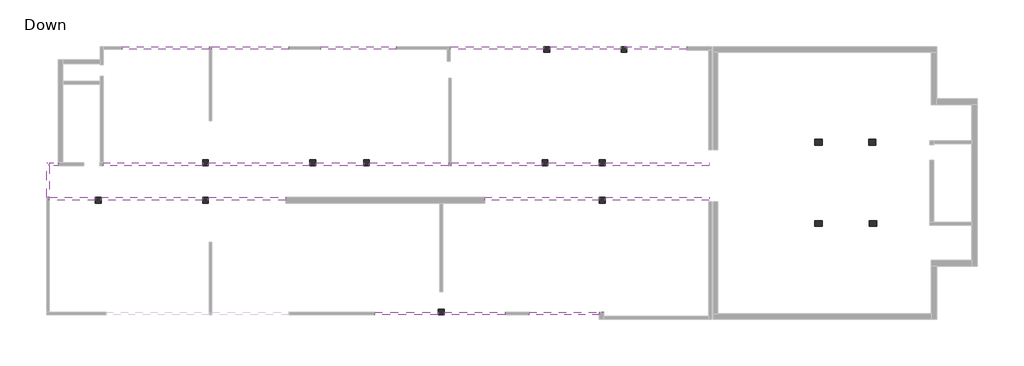
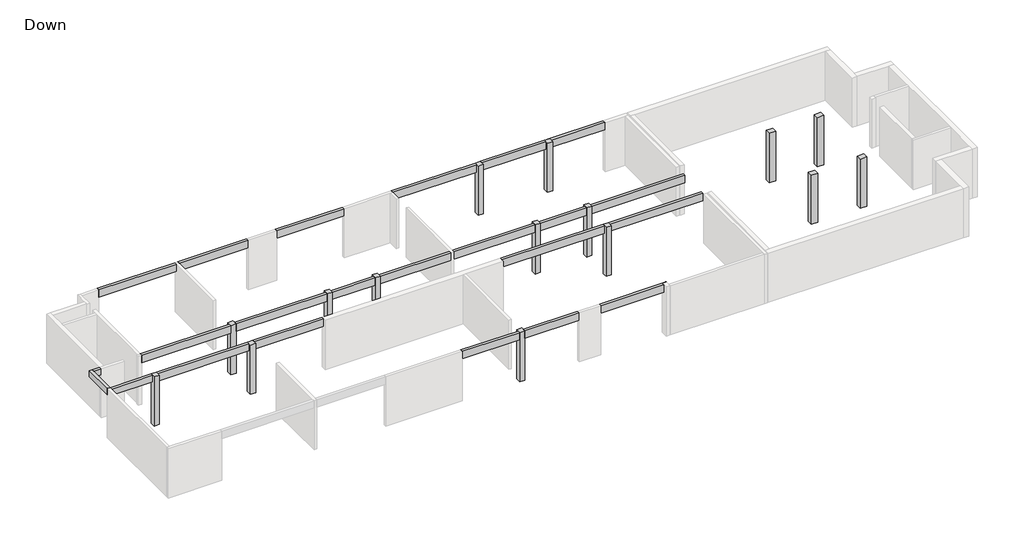
# One storey, part 2 of 2: 23 beams, 15 columns.
"""IFC4 building model written with IfcOpenShell, lengths in millimetres."""

from ifc_helpers import new_model, si_unit, origin, place, context, project, spatial, faceted_brep, element, save

model = new_model("IFC4")

# Units and contexts
model_context = context("Model", 3, world=origin())
ifc_project = project(units=[si_unit("LENGTHUNIT", "METRE", prefix="MILLI")], contexts=[model_context])

# Site, building, storey
site = spatial("IfcSite", under=ifc_project)
building = spatial("IfcBuilding", under=site)
storey = spatial("IfcBuildingStorey", under=building, Name="Down", Elevation=0.0)

# Beams
placement = place(None, origin())
element("IfcBeam", 1, ObjectType="Concrete Rectengular Beam : 20/50", at=placement, inside=storey, context=model_context, shape_type="Brep", body=[
    faceted_brep([(-20537.3553255, 3625.8513439, 4000.0), (-20537.3553255, 3825.8513439, 4000.0), (-23692.1640837, 3825.8513439, 4000.0), (-23692.1640837, 3625.8513439, 4000.0), (-20537.3553255, 3625.8513439, 3500.0), (-20537.3553255, 3625.8513439, 3730.0), (-23692.1640837, 3625.8513439, 3730.0), (-23692.1640837, 3625.8513439, 3500.0), (-20537.3553255, 3825.8513439, 3500.0), (-23692.1640837, 3825.8513439, 3500.0), (-20537.3553255, 3825.8513439, 3730.0), (-23692.1640837, 3825.8513439, 3730.0)], [[[0, 1, 2, 3]], [[4, 5, 0, 3, 6, 7]], [[8, 4, 7, 9]], [[2, 1, 10, 8, 9, 11]], [[1, 0, 5, 4, 8, 10]], [[3, 2, 11, 9, 7, 6]]]),
])
element("IfcBeam", 2, ObjectType="Concrete Rectengular Beam : 20/50", at=placement, inside=storey, context=model_context, shape_type="Brep", body=[
    faceted_brep([(-23692.1640837, 6225.0407157, 4000.0), (-23892.1640837, 6225.0407157, 4000.0), (-23892.1640837, 3825.8513439, 4000.0), (-23692.1640837, 3825.8513439, 4000.0), (-23692.1640837, 6025.0407157, 4000.0), (-23692.1640837, 6225.0407157, 3500.0), (-23692.1640837, 3825.8513439, 3730.0), (-23692.1640837, 3825.8513439, 3500.0), (-23692.1640837, 6025.0407157, 3500.0), (-23892.1640837, 6225.0407157, 3500.0), (-23892.1640837, 3825.8513439, 3500.0)], [[[0, 1, 2, 3, 4]], [[5, 0, 4, 3, 6, 7, 8]], [[9, 5, 8, 7, 10]], [[1, 9, 10, 2]], [[3, 2, 10, 7, 6]], [[1, 0, 5, 9]]]),
])
element("IfcBeam", 3, ObjectType="Concrete Rectengular Beam : 20/50", at=placement, inside=storey, context=model_context, shape_type="Brep", body=[
    faceted_brep([(-23692.1640837, 6225.0407157, 4000.0), (-23692.1640837, 6025.0407157, 4000.0), (-23092.0740139, 6025.0407157, 4000.0), (-23092.0740139, 6225.0407157, 4000.0), (-23692.1640837, 6025.0407157, 3730.0), (-23692.1640837, 6025.0407157, 3500.0), (-23092.0740139, 6025.0407157, 3500.0), (-23092.0740139, 6025.0407157, 3730.0), (-23692.1640837, 6225.0407157, 3500.0), (-23092.0740139, 6225.0407157, 3500.0)], [[[0, 1, 2, 3]], [[2, 1, 4, 5, 6, 7]], [[5, 8, 9, 6]], [[8, 0, 3, 9]], [[1, 0, 8, 5, 4]], [[3, 2, 7, 6, 9]]]),
])
element("IfcBeam", 4, ObjectType="Concrete Rectengular Beam : 20/65", at=placement, inside=storey, context=model_context, shape_type="Brep", body=[
    faceted_brep([(-13141.7475108, 6025.0407157, 4000.0), (-13141.7475108, 6225.0407157, 4000.0), (-19991.1958333, 6225.0407157, 4000.0), (-19991.1958333, 6025.0407157, 4000.0), (-19991.1958333, 6025.0407157, 3730.0), (-19991.1958333, 6025.0407157, 3400.0), (-13141.7475108, 6025.0407157, 3400.0), (-13141.7475108, 6025.0407157, 3730.0), (-13141.7475108, 6225.0407157, 3400.0), (-19991.1958333, 6225.0407157, 3400.0), (-13141.7475108, 6225.0407157, 3730.0), (-19991.1958333, 6225.0407157, 3730.0)], [[[0, 1, 2, 3]], [[0, 3, 4, 5, 6, 7]], [[8, 6, 5, 9]], [[2, 1, 10, 8, 9, 11]], [[1, 0, 7, 6, 8, 10]], [[3, 2, 11, 9, 5, 4]]]),
])
element("IfcBeam", 5, ObjectType="Concrete Rectengular Beam : 20/65", at=placement, inside=storey, context=model_context, shape_type="Brep", body=[
    faceted_brep([(-5741.9726853, 6025.0407157, 4000.0), (-5741.9726853, 6225.0407157, 4000.0), (-12741.7475108, 6225.0407157, 4000.0), (-12741.7475108, 6025.0407157, 4000.0), (-12741.7475108, 6025.0407157, 3730.0), (-12741.7475108, 6025.0407157, 3400.0), (-5741.9726853, 6025.0407157, 3400.0), (-5741.9726853, 6025.0407157, 3730.0), (-5741.9726853, 6225.0407157, 3400.0), (-12741.7475108, 6225.0407157, 3400.0), (-5741.9726853, 6225.0407157, 3730.0), (-12741.7475108, 6225.0407157, 3730.0)], [[[0, 1, 2, 3]], [[0, 3, 4, 5, 6, 7]], [[8, 6, 5, 9]], [[2, 1, 10, 8, 9, 11]], [[1, 0, 7, 6, 8, 10]], [[3, 2, 11, 9, 5, 4]]]),
])
element("IfcBeam", 6, ObjectType="Concrete Rectengular Beam : 20/65", at=placement, inside=storey, context=model_context, shape_type="Brep", body=[
    faceted_brep([(-2042.0852726, 6025.0407157, 4000.0), (-2042.0852726, 6225.0407157, 4000.0), (-5341.9726853, 6225.0407157, 4000.0), (-5341.9726853, 6025.0407157, 4000.0), (-5341.9726853, 6025.0407157, 3730.0), (-5341.9726853, 6025.0407157, 3400.0), (-2042.0852726, 6025.0407157, 3400.0), (-2042.0852726, 6025.0407157, 3730.0), (-2042.0852726, 6225.0407157, 3400.0), (-5341.9726853, 6225.0407157, 3400.0), (-2042.0852726, 6225.0407157, 3730.0), (-5341.9726853, 6225.0407157, 3730.0)], [[[0, 1, 2, 3]], [[0, 3, 4, 5, 6, 7]], [[8, 6, 5, 9]], [[2, 1, 10, 8, 9, 11]], [[1, 0, 7, 6, 8, 10]], [[3, 2, 11, 9, 5, 4]]]),
])
element("IfcBeam", 7, ObjectType="Concrete Rectengular Beam : 20/65", at=placement, inside=storey, context=model_context, shape_type="Brep", body=[
    faceted_brep([(-1642.0852726, 6225.0407157, 4000.0), (-1642.0852726, 6025.0407157, 4000.0), (3809.3896205, 6025.0407157, 4000.0), (3809.3896205, 6225.0407157, 4000.0), (-1642.0852726, 6025.0407157, 3730.0), (-1642.0852726, 6025.0407157, 3400.0), (3809.3896205, 6025.0407157, 3400.0), (3809.3896205, 6025.0407157, 3730.0), (-1642.0852726, 6225.0407157, 3400.0), (3809.3896205, 6225.0407157, 3400.0), (3809.3896205, 6225.0407157, 3730.0), (-1642.0852726, 6225.0407157, 3730.0)], [[[0, 1, 2, 3]], [[2, 1, 4, 5, 6, 7]], [[5, 8, 9, 6]], [[0, 3, 10, 9, 8, 11]], [[1, 0, 11, 8, 5, 4]], [[3, 2, 7, 6, 9, 10]]]),
])
element("IfcBeam", 8, ObjectType="Concrete Rectengular Beam : 20/65", at=placement, inside=storey, context=model_context, shape_type="Brep", body=[
    faceted_brep([(10255.59543, 6025.0407157, 4000.0), (10255.59543, 6225.0407157, 4000.0), (4009.3896205, 6225.0407157, 4000.0), (4009.3896205, 6025.0407157, 4000.0), (4009.3896205, 6025.0407157, 3730.0), (4009.3896205, 6025.0407157, 3400.0), (10255.59543, 6025.0407157, 3400.0), (10255.59543, 6025.0407157, 3730.0), (10255.59543, 6225.0407157, 3400.0), (4009.3896205, 6225.0407157, 3400.0), (10255.59543, 6225.0407157, 3730.0), (4009.3896205, 6225.0407157, 3730.0)], [[[0, 1, 2, 3]], [[0, 3, 4, 5, 6, 7]], [[8, 6, 5, 9]], [[2, 1, 10, 8, 9, 11]], [[1, 0, 7, 6, 8, 10]], [[3, 2, 11, 9, 5, 4]]]),
])
element("IfcBeam", 9, ObjectType="Concrete Rectengular Beam : 20/65", at=placement, inside=storey, context=model_context, shape_type="Brep", body=[
    faceted_brep([(10655.59543, 6225.0407157, 4000.0), (10655.59543, 6025.0407157, 4000.0), (14207.3630499, 6025.0407157, 4000.0), (14207.3630499, 6225.0407157, 4000.0), (10655.59543, 6025.0407157, 3730.0), (10655.59543, 6025.0407157, 3400.0), (14207.3630499, 6025.0407157, 3400.0), (14207.3630499, 6025.0407157, 3730.0), (10655.59543, 6225.0407157, 3400.0), (14207.3630499, 6225.0407157, 3400.0), (14207.3630499, 6225.0407157, 3730.0), (10655.59543, 6225.0407157, 3730.0)], [[[0, 1, 2, 3]], [[2, 1, 4, 5, 6, 7]], [[5, 8, 9, 6]], [[0, 3, 10, 9, 8, 11]], [[1, 0, 11, 8, 5, 4]], [[3, 2, 7, 6, 9, 10]]]),
])
element("IfcBeam", 10, ObjectType="Concrete Rectengular Beam : 20/65", at=placement, inside=storey, context=model_context, shape_type="Brep", body=[
    faceted_brep([(21767.3630499, 6025.0407157, 3400.0), (21767.3630499, 6225.0407157, 3400.0), (21767.3630499, 6225.0407157, 3730.0), (21767.3630499, 6225.0407157, 4000.0), (21767.3630499, 6129.9270025, 4000.0), (21767.3630499, 6025.0407157, 4000.0), (21767.3630499, 6025.0407157, 3730.0), (14607.3630499, 6225.0407157, 4000.0), (14607.3630499, 6025.0407157, 4000.0), (14607.3630499, 6025.0407157, 3730.0), (14607.3630499, 6025.0407157, 3400.0), (14607.3630499, 6225.0407157, 3400.0), (14607.3630499, 6225.0407157, 3730.0)], [[[0, 1, 2, 3, 4, 5, 6]], [[3, 7, 8, 5, 4]], [[5, 8, 9, 10, 0, 6]], [[1, 0, 10, 11]], [[7, 3, 2, 1, 11, 12]], [[8, 7, 12, 11, 10, 9]]]),
])
element("IfcBeam", 11, ObjectType="Concrete Rectengular Beam : 20/65", at=placement, inside=storey, context=model_context, shape_type="Brep", body=[
    faceted_brep([(-20137.3553255, 3825.8513439, 4000.0), (-20137.3553255, 3625.8513439, 4000.0), (-13141.7475108, 3625.8513439, 4000.0), (-13141.7475108, 3825.8513439, 4000.0), (-20137.3553255, 3625.8513439, 3730.0), (-20137.3553255, 3625.8513439, 3400.0), (-13141.7475108, 3625.8513439, 3400.0), (-13141.7475108, 3625.8513439, 3730.0), (-20137.3553255, 3825.8513439, 3400.0), (-13141.7475108, 3825.8513439, 3400.0), (-13141.7475108, 3825.8513439, 3730.0), (-20137.3553255, 3825.8513439, 3730.0)], [[[0, 1, 2, 3]], [[1, 4, 5, 6, 7, 2]], [[5, 8, 9, 6]], [[0, 3, 10, 9, 8, 11]], [[1, 0, 11, 8, 5, 4]], [[3, 2, 7, 6, 9, 10]]]),
])
element("IfcBeam", 12, ObjectType="Concrete Rectengular Beam : 20/65", at=placement, inside=storey, context=model_context, shape_type="Brep", body=[
    faceted_brep([(-12741.7475108, 3825.8513439, 4000.0), (-12741.7475108, 3625.8513439, 4000.0), (-7390.8355541, 3625.8513439, 4000.0), (-7390.8355541, 3825.8513439, 4000.0), (-12741.7475108, 3625.8513439, 3730.0), (-12741.7475108, 3625.8513439, 3400.0), (-7390.8355541, 3625.8513439, 3400.0), (-7390.8355541, 3625.8513439, 3730.0), (-12741.7475108, 3825.8513439, 3400.0), (-7390.8355541, 3825.8513439, 3400.0), (-7390.8355541, 3825.8513439, 3730.0), (-12741.7475108, 3825.8513439, 3730.0)], [[[0, 1, 2, 3]], [[1, 4, 5, 6, 7, 2]], [[5, 8, 9, 6]], [[0, 3, 10, 9, 8, 11]], [[1, 0, 11, 8, 5, 4]], [[3, 2, 7, 6, 9, 10]]]),
])
element("IfcBeam", 13, ObjectType="Concrete Rectengular Beam : 20/65", at=placement, inside=storey, context=model_context, shape_type="Brep", body=[
    faceted_brep([(14207.3630499, 3625.8513439, 4000.0), (14207.3630499, 3825.8513439, 4000.0), (6309.1644459, 3825.8513439, 4000.0), (6309.1644459, 3625.8513439, 4000.0), (14207.3630499, 3825.8513439, 3730.0), (14207.3630499, 3825.8513439, 3400.0), (6309.1644459, 3825.8513439, 3400.0), (6309.1644459, 3825.8513439, 3730.0), (14207.3630499, 3625.8513439, 3400.0), (6309.1644459, 3625.8513439, 3400.0), (14207.3630499, 3625.8513439, 3730.0), (6309.1644459, 3625.8513439, 3730.0)], [[[0, 1, 2, 3]], [[2, 1, 4, 5, 6, 7]], [[5, 8, 9, 6]], [[8, 10, 0, 3, 11, 9]], [[8, 5, 4, 1, 0, 10]], [[6, 9, 11, 3, 2, 7]]]),
])
element("IfcBeam", 14, ObjectType="Concrete Rectengular Beam : 20/65", at=placement, inside=storey, context=model_context, shape_type="Brep", body=[
    faceted_brep([(21767.3630499, 3825.8513439, 4000.0), (21767.3630499, 3625.8513439, 4000.0), (21767.3630499, 3625.8513439, 3730.0), (21767.3630499, 3625.8513439, 3400.0), (21767.3630499, 3825.8513439, 3400.0), (21767.3630499, 3825.8513439, 3730.0), (14607.3630499, 3825.8513439, 4000.0), (14607.3630499, 3625.8513439, 4000.0), (21760.6168215, 3625.8513439, 4000.0), (14607.3630499, 3625.8513439, 3400.0), (14607.3630499, 3625.8513439, 3730.0), (14607.3630499, 3825.8513439, 3400.0), (14607.3630499, 3825.8513439, 3730.0)], [[[0, 1, 2, 3, 4, 5]], [[1, 0, 6, 7, 8]], [[9, 3, 2, 1, 8, 7, 10]], [[4, 3, 9, 11]], [[4, 11, 12, 6, 0, 5]], [[9, 10, 7, 6, 12, 11]]]),
])
element("IfcBeam", 15, ObjectType="Concrete Rectengular Beam : 20/65", at=placement, inside=storey, context=model_context, shape_type="Brep", body=[
    faceted_brep([(-1290.6779319, -4074.5314528, 4000.0), (-1290.6779319, -4274.5314528, 4000.0), (3109.817452, -4274.5314528, 4000.0), (3109.817452, -4074.5314528, 4000.0), (-1290.6779319, -4274.5314528, 3400.0), (3109.817452, -4274.5314528, 3400.0), (-1290.6779319, -4074.5314528, 3400.0), (3109.817452, -4074.5314528, 3400.0), (3109.817452, -4074.5314528, 3730.0), (-1290.6779319, -4074.5314528, 3730.0)], [[[0, 1, 2, 3]], [[1, 4, 5, 2]], [[4, 6, 7, 5]], [[0, 3, 8, 7, 6, 9]], [[4, 1, 0, 9, 6]], [[3, 2, 5, 7, 8]]]),
])
element("IfcBeam", 16, ObjectType="Concrete Rectengular Beam : 20/65", at=placement, inside=storey, context=model_context, shape_type="Brep", body=[
    faceted_brep([(3509.817452, -4074.5314528, 4000.0), (3509.817452, -4274.5314528, 4000.0), (7709.2770332, -4274.5314528, 4000.0), (7709.2770332, -4074.5314528, 4000.0), (3509.817452, -4274.5314528, 3400.0), (7709.2770332, -4274.5314528, 3400.0), (3509.817452, -4074.5314528, 3400.0), (7709.2770332, -4074.5314528, 3400.0), (7709.2770332, -4074.5314528, 3730.0), (3509.817452, -4074.5314528, 3730.0)], [[[0, 1, 2, 3]], [[1, 4, 5, 2]], [[4, 6, 7, 5]], [[0, 3, 8, 7, 6, 9]], [[1, 0, 9, 6, 4]], [[3, 2, 5, 7, 8]]]),
])
element("IfcBeam", 17, ObjectType="Concrete Rectengular Beam : 20/65", at=placement, inside=storey, context=model_context, shape_type="Brep", body=[
    faceted_brep([(14509.4796903, -4075.5672555, 4000.0), (14509.4796903, -4074.5314528, 4000.0), (9358.1399019, -4074.5314528, 4000.0), (9358.1399019, -4274.5314528, 4000.0), (14209.4796903, -4274.5314528, 4000.0), (14209.4796903, -4075.5672555, 4000.0), (14209.4796903, -4274.5314528, 3400.0), (9358.1399019, -4274.5314528, 3400.0), (14509.4796903, -4074.5314528, 3400.0), (14509.4796903, -4075.5672555, 3400.0), (14209.4796903, -4075.5672555, 3400.0), (9358.1399019, -4074.5314528, 3400.0), (14509.4796903, -4074.5314528, 3730.0), (9358.1399019, -4074.5314528, 3730.0), (14509.4796903, -4075.5672555, 3730.0)], [[[0, 1, 2, 3, 4, 5]], [[6, 4, 3, 7]], [[8, 9, 10, 6, 7, 11]], [[2, 1, 12, 8, 11, 13]], [[1, 0, 14, 9, 8, 12]], [[10, 5, 4, 6]], [[5, 10, 9, 14, 0]], [[3, 2, 13, 11, 7]]]),
])
element("IfcBeam", 18, ObjectType="Concrete Rectengular Beam : 20/65", at=placement, inside=storey, context=model_context, shape_type="Brep", body=[
    faceted_brep([(-12690.9031064, 14024.905611, 4000.0), (-12690.9031064, 14224.905611, 4000.0), (-18691.5786299, 14224.905611, 4000.0), (-18691.5786299, 14024.905611, 4000.0), (-18691.5786299, 14024.905611, 3730.0), (-18691.5786299, 14024.905611, 3400.0), (-12690.9031064, 14024.905611, 3400.0), (-12690.9031064, 14024.905611, 3730.0), (-12690.9031064, 14224.905611, 3400.0), (-18691.5786299, 14224.905611, 3400.0)], [[[0, 1, 2, 3]], [[0, 3, 4, 5, 6, 7]], [[8, 6, 5, 9]], [[1, 8, 9, 2]], [[1, 0, 7, 6, 8]], [[3, 2, 9, 5, 4]]]),
])
element("IfcBeam", 19, ObjectType="Concrete Rectengular Beam : 20/65", at=placement, inside=storey, context=model_context, shape_type="Brep", body=[
    faceted_brep([(-12490.9031064, 14224.905611, 4000.0), (-12490.9031064, 14024.905611, 4000.0), (-7191.8713568, 14024.905611, 4000.0), (-7191.8713568, 14224.905611, 4000.0), (-12490.9031064, 14024.905611, 3730.0), (-12490.9031064, 14024.905611, 3400.0), (-7191.8713568, 14024.905611, 3400.0), (-7191.8713568, 14024.905611, 3730.0), (-12490.9031064, 14224.905611, 3400.0), (-7191.8713568, 14224.905611, 3400.0)], [[[0, 1, 2, 3]], [[2, 1, 4, 5, 6, 7]], [[5, 8, 9, 6]], [[8, 0, 3, 9]], [[1, 0, 8, 5, 4]], [[3, 2, 7, 6, 9]]]),
])
element("IfcBeam", 20, ObjectType="Concrete Rectengular Beam : 20/65", at=placement, inside=storey, context=model_context, shape_type="Brep", body=[
    faceted_brep([(-4990.5653446, 14224.905611, 4000.0), (-4990.5653446, 14024.905611, 4000.0), (207.9034687, 14024.905611, 4000.0), (207.9034687, 14224.905611, 4000.0), (-4990.5653446, 14024.905611, 3730.0), (-4990.5653446, 14024.905611, 3400.0), (207.9034687, 14024.905611, 3400.0), (207.9034687, 14024.905611, 3730.0), (-4990.5653446, 14224.905611, 3400.0), (207.9034687, 14224.905611, 3400.0)], [[[0, 1, 2, 3]], [[2, 1, 4, 5, 6, 7]], [[5, 8, 9, 6]], [[3, 9, 8, 0]], [[1, 0, 8, 5, 4]], [[3, 2, 7, 6, 9]]]),
])
element("IfcBeam", 21, ObjectType="Concrete Rectengular Beam : 20/65", at=placement, inside=storey, context=model_context, shape_type="Brep", body=[
    faceted_brep([(10383.8278101, 14024.905611, 4000.0), (10383.8278101, 14224.905611, 4000.0), (3933.1905662, 14224.905611, 4000.0), (3933.1905662, 14024.905611, 4000.0), (3933.1905662, 14024.905611, 3730.0), (3933.1905662, 14024.905611, 3400.0), (10383.8278101, 14024.905611, 3400.0), (10383.8278101, 14024.905611, 3730.0), (10383.8278101, 14224.905611, 3400.0), (3933.1905662, 14224.905611, 3400.0)], [[[0, 1, 2, 3]], [[0, 3, 4, 5, 6, 7]], [[8, 6, 5, 9]], [[1, 8, 9, 2]], [[1, 0, 7, 6, 8]], [[3, 2, 9, 5, 4]]]),
])
element("IfcBeam", 22, ObjectType="Concrete Rectengular Beam : 20/65", at=placement, inside=storey, context=model_context, shape_type="Brep", body=[
    faceted_brep([(15703.8278101, 14024.905611, 4000.0), (15703.8278101, 14224.905611, 4000.0), (10783.8278101, 14224.905611, 4000.0), (10783.8278101, 14024.905611, 4000.0), (10783.8278101, 14024.905611, 3730.0), (10783.8278101, 14024.905611, 3400.0), (15703.8278101, 14024.905611, 3400.0), (15703.8278101, 14024.905611, 3730.0), (15703.8278101, 14224.905611, 3400.0), (10783.8278101, 14224.905611, 3400.0)], [[[0, 1, 2, 3]], [[0, 3, 4, 5, 6, 7]], [[8, 6, 5, 9]], [[1, 8, 9, 2]], [[1, 0, 7, 6, 8]], [[3, 2, 9, 5, 4]]]),
])
element("IfcBeam", 23, ObjectType="Concrete Rectengular Beam : 20/65", at=placement, inside=storey, context=model_context, shape_type="Brep", body=[
    faceted_brep([(16103.8278101, 14224.905611, 4000.0), (16103.8278101, 14025.1420442, 4000.0), (20235.5548985, 14025.1420442, 4000.0), (20235.5548985, 14225.1420442, 4000.0), (15903.8278101, 14225.1420442, 4000.0), (15903.8278101, 14224.905611, 4000.0), (16103.8278101, 14025.1420442, 3730.0), (16103.8278101, 14025.1420442, 3400.0), (20235.5548985, 14025.1420442, 3400.0), (20235.5548985, 14025.1420442, 3730.0), (16103.8278101, 14224.905611, 3400.0), (15903.8278101, 14224.905611, 3400.0), (15903.8278101, 14225.1420442, 3400.0), (20235.5548985, 14225.1420442, 3400.0)], [[[0, 1, 2, 3, 4, 5]], [[1, 6, 7, 8, 9, 2]], [[7, 10, 11, 12, 13, 8]], [[12, 4, 3, 13]], [[4, 12, 11, 5]], [[1, 0, 10, 7, 6]], [[3, 2, 9, 8, 13]], [[10, 0, 5, 11]]]),
])

# Columns
element("IfcColumn", 24, ObjectType="Concrete Rectengular Column : 40/40", at=placement, inside=storey, context=model_context, shape_type="Brep", body=[
    faceted_brep([(-20137.3553255, 3825.8513439, 0.0), (-20137.3553255, 3425.8513439, 0.0), (-20537.3553255, 3425.8513439, 0.0), (-20537.3553255, 3825.8513439, 0.0), (-20137.3553255, 3825.8513439, 4000.0), (-20137.3553255, 3625.8513439, 4000.0), (-20137.3553255, 3425.8513439, 4000.0), (-20137.3553255, 3425.8513439, 3730.0), (-20537.3553255, 3425.8513439, 4000.0), (-20537.3553255, 3425.8513439, 3730.0), (-20537.3553255, 3625.8513439, 4000.0), (-20537.3553255, 3825.8513439, 4000.0)], [[[0, 1, 2, 3]], [[4, 5, 6, 7, 1, 0]], [[6, 8, 9, 2, 1, 7]], [[8, 10, 11, 3, 2, 9]], [[11, 4, 0, 3]], [[4, 11, 10, 8, 6, 5]]]),
])
element("IfcColumn", 25, ObjectType="Concrete Rectengular Column : 40/40", at=placement, inside=storey, context=model_context, shape_type="Brep", body=[
    faceted_brep([(16103.8278101, 14224.905611, 0.0), (16103.8278101, 13824.905611, 0.0), (15703.8278101, 13824.905611, 0.0), (15703.8278101, 14224.905611, 0.0), (16103.8278101, 14224.905611, 4000.0), (16103.8278101, 14025.1420442, 4000.0), (16103.8278101, 13824.905611, 4000.0), (16103.8278101, 13824.905611, 3730.0), (15703.8278101, 13824.905611, 4000.0), (15703.8278101, 13824.905611, 3730.0), (15703.8278101, 14024.905611, 4000.0), (15703.8278101, 14224.905611, 4000.0)], [[[0, 1, 2, 3]], [[4, 5, 6, 7, 1, 0]], [[6, 8, 9, 2, 1, 7]], [[8, 10, 11, 3, 2, 9]], [[11, 4, 0, 3]], [[4, 11, 10, 8, 6, 5]]]),
])
element("IfcColumn", 26, ObjectType="Concrete Rectengular Column : 40/40", at=placement, inside=storey, context=model_context, shape_type="Brep", body=[
    faceted_brep([(10783.8278101, 14224.905611, 0.0), (10783.8278101, 13824.905611, 0.0), (10383.8278101, 13824.905611, 0.0), (10383.8278101, 14224.905611, 0.0), (10783.8278101, 14224.905611, 4000.0), (10783.8278101, 14024.905611, 4000.0), (10783.8278101, 13824.905611, 4000.0), (10783.8278101, 13824.905611, 3730.0), (10383.8278101, 13824.905611, 4000.0), (10383.8278101, 13824.905611, 3730.0), (10383.8278101, 14024.905611, 4000.0), (10383.8278101, 14224.905611, 4000.0)], [[[0, 1, 2, 3]], [[4, 5, 6, 7, 1, 0]], [[6, 8, 9, 2, 1, 7]], [[8, 10, 11, 3, 2, 9]], [[11, 4, 0, 3]], [[4, 11, 10, 8, 6, 5]]]),
])
element("IfcColumn", 27, ObjectType="Concrete Rectengular Column : 40/40", at=placement, inside=storey, context=model_context, shape_type="Brep", body=[
    faceted_brep([(10655.59543, 6425.0407157, 0.0), (10655.59543, 6025.0407157, 0.0), (10255.59543, 6025.0407157, 0.0), (10255.59543, 6425.0407157, 0.0), (10655.59543, 6425.0407157, 4000.0), (10655.59543, 6225.0407157, 4000.0), (10655.59543, 6025.0407157, 4000.0), (10655.59543, 6425.0407157, 3730.0), (10255.59543, 6025.0407157, 4000.0), (10255.59543, 6225.0407157, 4000.0), (10255.59543, 6425.0407157, 4000.0), (10255.59543, 6425.0407157, 3730.0)], [[[0, 1, 2, 3]], [[4, 5, 6, 1, 0, 7]], [[6, 8, 2, 1]], [[8, 9, 10, 11, 3, 2]], [[10, 4, 7, 0, 3, 11]], [[4, 10, 9, 8, 6, 5]]]),
])
element("IfcColumn", 28, ObjectType="Concrete Rectengular Column : 40/40", at=placement, inside=storey, context=model_context, shape_type="Brep", body=[
    faceted_brep([(14607.3630499, 6425.0407157, 0.0), (14607.3630499, 6025.0407157, 0.0), (14207.3630499, 6025.0407157, 0.0), (14207.3630499, 6425.0407157, 0.0), (14607.3630499, 6425.0407157, 4000.0), (14607.3630499, 6225.0407157, 4000.0), (14607.3630499, 6025.0407157, 4000.0), (14607.3630499, 6425.0407157, 3730.0), (14207.3630499, 6025.0407157, 4000.0), (14207.3630499, 6225.0407157, 4000.0), (14207.3630499, 6425.0407157, 4000.0), (14207.3630499, 6425.0407157, 3730.0)], [[[0, 1, 2, 3]], [[4, 5, 6, 1, 0, 7]], [[6, 8, 2, 1]], [[8, 9, 10, 11, 3, 2]], [[10, 4, 7, 0, 3, 11]], [[4, 10, 9, 8, 6, 5]]]),
])
element("IfcColumn", 29, ObjectType="Concrete Rectengular Column : 40/40", at=placement, inside=storey, context=model_context, shape_type="Brep", body=[
    faceted_brep([(14607.3630499, 3825.806309, 0.0), (14607.3630499, 3425.806309, 0.0), (14207.3630499, 3425.806309, 0.0), (14207.3630499, 3825.806309, 0.0), (14607.3630499, 3825.806309, 4000.0), (14607.3630499, 3625.8513439, 4000.0), (14607.3630499, 3425.806309, 4000.0), (14607.3630499, 3425.806309, 3730.0), (14207.3630499, 3425.806309, 4000.0), (14207.3630499, 3425.806309, 3730.0), (14207.3630499, 3625.806309, 4000.0), (14207.3630499, 3825.806309, 4000.0)], [[[0, 1, 2, 3]], [[4, 5, 6, 7, 1, 0]], [[6, 8, 9, 2, 1, 7]], [[8, 10, 11, 3, 2, 9]], [[11, 4, 0, 3]], [[4, 11, 10, 8, 6, 5]]]),
])
element("IfcColumn", 30, ObjectType="Concrete Rectengular Column : 40/40", at=placement, inside=storey, context=model_context, shape_type="Brep", body=[
    faceted_brep([(-1642.0852726, 6425.0407157, 0.0), (-1642.0852726, 6025.0407157, 0.0), (-2042.0852726, 6025.0407157, 0.0), (-2042.0852726, 6425.0407157, 0.0), (-1642.0852726, 6425.0407157, 4000.0), (-1642.0852726, 6225.0407157, 4000.0), (-1642.0852726, 6025.0407157, 4000.0), (-1642.0852726, 6425.0407157, 3730.0), (-2042.0852726, 6025.0407157, 4000.0), (-2042.0852726, 6225.0407157, 4000.0), (-2042.0852726, 6425.0407157, 4000.0), (-2042.0852726, 6425.0407157, 3730.0)], [[[0, 1, 2, 3]], [[4, 5, 6, 1, 0, 7]], [[6, 8, 2, 1]], [[8, 9, 10, 11, 3, 2]], [[10, 4, 7, 0, 3, 11]], [[4, 10, 9, 8, 6, 5]]]),
])
element("IfcColumn", 31, ObjectType="Concrete Rectengular Column : 40/40", at=placement, inside=storey, context=model_context, shape_type="Brep", body=[
    faceted_brep([(-5341.9726853, 6425.0407157, 0.0), (-5341.9726853, 6025.0407157, 0.0), (-5741.9726853, 6025.0407157, 0.0), (-5741.9726853, 6425.0407157, 0.0), (-5341.9726853, 6425.0407157, 4000.0), (-5341.9726853, 6225.0407157, 4000.0), (-5341.9726853, 6025.0407157, 4000.0), (-5341.9726853, 6425.0407157, 3730.0), (-5741.9726853, 6025.0407157, 4000.0), (-5741.9726853, 6225.0407157, 4000.0), (-5741.9726853, 6425.0407157, 4000.0), (-5741.9726853, 6425.0407157, 3730.0)], [[[0, 1, 2, 3]], [[4, 5, 6, 1, 0, 7]], [[6, 8, 2, 1]], [[8, 9, 10, 11, 3, 2]], [[10, 4, 7, 0, 3, 11]], [[4, 10, 9, 8, 6, 5]]]),
])
element("IfcColumn", 32, ObjectType="Concrete Rectengular Column : 40/40", at=placement, inside=storey, context=model_context, shape_type="Brep", body=[
    faceted_brep([(-12741.7475108, 6425.0407157, 0.0), (-12741.7475108, 6025.0407157, 0.0), (-13141.7475108, 6025.0407157, 0.0), (-13141.7475108, 6425.0407157, 0.0), (-12741.7475108, 6425.0407157, 4000.0), (-12741.7475108, 6225.0407157, 4000.0), (-12741.7475108, 6025.0407157, 4000.0), (-12741.7475108, 6425.0407157, 3730.0), (-13141.7475108, 6025.0407157, 4000.0), (-13141.7475108, 6225.0407157, 4000.0), (-13141.7475108, 6425.0407157, 4000.0), (-13141.7475108, 6425.0407157, 3730.0)], [[[0, 1, 2, 3]], [[4, 5, 6, 1, 0, 7]], [[6, 8, 2, 1]], [[8, 9, 10, 11, 3, 2]], [[10, 4, 7, 0, 3, 11]], [[4, 10, 9, 8, 6, 5]]]),
])
element("IfcColumn", 33, ObjectType="Concrete Rectengular Column : 40/40", at=placement, inside=storey, context=model_context, shape_type="Brep", body=[
    faceted_brep([(-12741.7475108, 3825.806309, 0.0), (-12741.7475108, 3425.806309, 0.0), (-13141.7475108, 3425.806309, 0.0), (-13141.7475108, 3825.806309, 0.0), (-12741.7475108, 3825.806309, 4000.0), (-12741.7475108, 3625.806309, 4000.0), (-12741.7475108, 3425.806309, 4000.0), (-12741.7475108, 3425.806309, 3730.0), (-13141.7475108, 3425.806309, 4000.0), (-13141.7475108, 3425.806309, 3730.0), (-13141.7475108, 3625.8513439, 4000.0), (-13141.7475108, 3825.806309, 4000.0)], [[[0, 1, 2, 3]], [[4, 5, 6, 7, 1, 0]], [[6, 8, 9, 2, 1, 7]], [[8, 10, 11, 3, 2, 9]], [[11, 4, 0, 3]], [[4, 11, 10, 8, 6, 5]]]),
])
element("IfcColumn", 34, ObjectType="Concrete Rectengular Column : 40/40", at=placement, inside=storey, context=model_context, shape_type="Brep", body=[
    faceted_brep([(3509.817452, -3874.5314528, 0.0), (3509.817452, -4274.5314528, 0.0), (3109.817452, -4274.5314528, 0.0), (3109.817452, -3874.5314528, 0.0), (3509.817452, -3874.5314528, 4000.0), (3509.817452, -4074.5314528, 4000.0), (3509.817452, -4274.5314528, 4000.0), (3509.817452, -3874.5314528, 3730.0), (3109.817452, -4274.5314528, 4000.0), (3109.817452, -4274.5314528, 3400.0), (3109.817452, -4074.5314528, 4000.0), (3109.817452, -3874.5314528, 4000.0), (3109.817452, -3874.5314528, 3730.0)], [[[0, 1, 2, 3]], [[4, 5, 6, 1, 0, 7]], [[6, 8, 9, 2, 1]], [[8, 10, 11, 12, 3, 2, 9]], [[11, 4, 7, 0, 3, 12]], [[4, 11, 10, 8, 6, 5]]]),
])
element("IfcColumn", 35, ObjectType="Concrete Rectengular Column : 40/50", at=placement, inside=storey, context=model_context, shape_type="Brep", body=[
    faceted_brep([(29059.8287108, 7824.1850525, 0.0), (29559.8287108, 7824.1850525, 0.0), (29559.8287108, 7424.1850525, 0.0), (29059.8287108, 7424.1850525, 0.0), (29059.8287108, 7824.1850525, 4000.0), (29559.8287108, 7824.1850525, 4000.0), (29559.8287108, 7824.1850525, 3730.0), (29059.8287108, 7824.1850525, 3730.0), (29559.8287108, 7424.1850525, 4000.0), (29559.8287108, 7424.1850525, 3730.0), (29059.8287108, 7424.1850525, 4000.0), (29059.8287108, 7424.1850525, 3730.0)], [[[0, 1, 2, 3]], [[4, 5, 6, 1, 0, 7]], [[5, 8, 9, 2, 1, 6]], [[8, 10, 11, 3, 2, 9]], [[10, 4, 7, 0, 3, 11]], [[4, 10, 8, 5]]]),
])
element("IfcColumn", 36, ObjectType="Concrete Rectengular Column : 40/50", at=placement, inside=storey, context=model_context, shape_type="Brep", body=[
    faceted_brep([(32759.8287108, 7824.1850525, 0.0), (33259.8287108, 7824.1850525, 0.0), (33259.8287108, 7424.1850525, 0.0), (32759.8287108, 7424.1850525, 0.0), (32759.8287108, 7824.1850525, 4000.0), (33259.8287108, 7824.1850525, 4000.0), (33259.8287108, 7824.1850525, 3730.0), (32759.8287108, 7824.1850525, 3730.0), (33259.8287108, 7424.1850525, 4000.0), (33259.8287108, 7424.1850525, 3730.0), (32759.8287108, 7424.1850525, 4000.0), (32759.8287108, 7424.1850525, 3730.0)], [[[0, 1, 2, 3]], [[4, 5, 6, 1, 0, 7]], [[5, 8, 9, 2, 1, 6]], [[8, 10, 11, 3, 2, 9]], [[10, 4, 7, 0, 3, 11]], [[4, 10, 8, 5]]]),
])
element("IfcColumn", 37, ObjectType="Concrete Rectengular Column : 40/50", at=placement, inside=storey, context=model_context, shape_type="Brep", body=[
    faceted_brep([(32812.1592669, 2225.6261694, 0.0), (33312.1592669, 2225.6261694, 0.0), (33312.1592669, 1825.6261694, 0.0), (32812.1592669, 1825.6261694, 0.0), (32812.1592669, 2225.6261694, 4000.0), (33312.1592669, 2225.6261694, 4000.0), (33312.1592669, 2225.6261694, 3730.0), (32812.1592669, 2225.6261694, 3730.0), (33312.1592669, 1825.6261694, 4000.0), (33312.1592669, 1825.6261694, 3730.0), (32812.1592669, 1825.6261694, 4000.0), (32812.1592669, 1825.6261694, 3730.0)], [[[0, 1, 2, 3]], [[4, 5, 6, 1, 0, 7]], [[5, 8, 9, 2, 1, 6]], [[8, 10, 11, 3, 2, 9]], [[10, 4, 7, 0, 3, 11]], [[4, 10, 8, 5]]]),
])
element("IfcColumn", 38, ObjectType="Concrete Rectengular Column : 40/50", at=placement, inside=storey, context=model_context, shape_type="Brep", body=[
    faceted_brep([(29059.8287108, 2225.6261694, 0.0), (29559.8287108, 2225.6261694, 0.0), (29559.8287108, 1825.6261694, 0.0), (29059.8287108, 1825.6261694, 0.0), (29059.8287108, 2225.6261694, 4000.0), (29559.8287108, 2225.6261694, 4000.0), (29559.8287108, 2225.6261694, 3730.0), (29059.8287108, 2225.6261694, 3730.0), (29559.8287108, 1825.6261694, 4000.0), (29559.8287108, 1825.6261694, 3730.0), (29059.8287108, 1825.6261694, 4000.0), (29059.8287108, 1825.6261694, 3730.0)], [[[0, 1, 2, 3]], [[4, 5, 6, 1, 0, 7]], [[5, 8, 9, 2, 1, 6]], [[8, 10, 11, 3, 2, 9]], [[10, 4, 7, 0, 3, 11]], [[4, 10, 8, 5]]]),
])

save(model, "model.ifc")

# Revit data of these elements
# Type "Concrete Rectengular Beam : 20/50"
#   Length [instance default] = 152.4 cm
#   b = 20 cm
#   h = 50 cm
#   Structural Material [instance default] = Concrete
#   Assembly Code = ""
# Type "Concrete Rectengular Beam : 20/65"
#   Length [instance default] = 152.4 cm
#   b = 20 cm
#   h = 60 cm
#   Structural Material [instance default] = Concrete
#   Assembly Code = ""
# Type "Concrete Rectengular Column : 40/40"
#   b = 40 cm
#   h = 40 cm
#   Structural Material [instance default] = Concrete
# Type "Concrete Rectengular Column : 40/50"
#   b = 40 cm
#   h = 50 cm
#   Structural Material [instance default] = Concrete
# Element 1 (IfcBeam, "Concrete Rectengular Beam : 20/50")
#   Comments = ""
#   Mark = "B1"
#   SOFiSTiK_AMG_Comments = ""
#   SOFiSTiK_AMG_Scheduled = yes
#   SOFiSTiK_AMG_Adjusted = yes
#   Structural Material = Concrete
#   Phase Created = New Construction
#   Materials on its faces: "Concrete"
# Element 2 (IfcBeam, "Concrete Rectengular Beam : 20/50")
#   Comments = ""
#   Mark = "B2"
#   SOFiSTiK_AMG_Comments = ""
#   SOFiSTiK_AMG_Scheduled = yes
#   SOFiSTiK_AMG_Adjusted = yes
#   Structural Material = Concrete
#   Phase Created = New Construction
#   Materials on its faces: "Concrete"
# Element 3 (IfcBeam, "Concrete Rectengular Beam : 20/50")
#   Comments = ""
#   Mark = "B3"
#   SOFiSTiK_AMG_Comments = ""
#   SOFiSTiK_AMG_Scheduled = yes
#   SOFiSTiK_AMG_Adjusted = yes
#   Structural Material = Concrete
#   Phase Created = New Construction
#   Materials on its faces: "Concrete"
# Element 4 (IfcBeam, "Concrete Rectengular Beam : 20/65")
#   Comments = ""
#   Mark = "B4"
#   SOFiSTiK_AMG_Comments = ""
#   SOFiSTiK_AMG_Scheduled = yes
#   SOFiSTiK_AMG_Adjusted = yes
#   Structural Material = Concrete
#   Phase Created = New Construction
#   Materials on its faces: "Concrete"
# Element 5 (IfcBeam, "Concrete Rectengular Beam : 20/65")
#   Comments = ""
#   Mark = "B5"
#   SOFiSTiK_AMG_Comments = ""
#   SOFiSTiK_AMG_Scheduled = yes
#   SOFiSTiK_AMG_Adjusted = yes
#   Structural Material = Concrete
#   Phase Created = New Construction
#   Materials on its faces: "Concrete"
# Element 6 (IfcBeam, "Concrete Rectengular Beam : 20/65")
#   Comments = ""
#   Mark = "B6"
#   SOFiSTiK_AMG_Comments = ""
#   SOFiSTiK_AMG_Scheduled = yes
#   SOFiSTiK_AMG_Adjusted = yes
#   Structural Material = Concrete
#   Phase Created = New Construction
#   Materials on its faces: "Concrete"
# Element 7 (IfcBeam, "Concrete Rectengular Beam : 20/65")
#   Comments = ""
#   Mark = "B7"
#   SOFiSTiK_AMG_Comments = ""
#   SOFiSTiK_AMG_Scheduled = yes
#   SOFiSTiK_AMG_Adjusted = yes
#   Structural Material = Concrete
#   Phase Created = New Construction
#   Materials on its faces: "Concrete"
# Element 8 (IfcBeam, "Concrete Rectengular Beam : 20/65")
#   Comments = ""
#   Mark = "B8"
#   SOFiSTiK_AMG_Comments = ""
#   SOFiSTiK_AMG_Scheduled = yes
#   SOFiSTiK_AMG_Adjusted = yes
#   Structural Material = Concrete
#   Phase Created = New Construction
#   Materials on its faces: "Concrete"
# Element 9 (IfcBeam, "Concrete Rectengular Beam : 20/65")
#   Comments = ""
#   Mark = "B9"
#   SOFiSTiK_AMG_Comments = ""
#   SOFiSTiK_AMG_Scheduled = yes
#   SOFiSTiK_AMG_Adjusted = yes
#   Structural Material = Concrete
#   Phase Created = New Construction
#   Materials on its faces: "Concrete"
# Element 10 (IfcBeam, "Concrete Rectengular Beam : 20/65")
#   Comments = ""
#   Mark = "B10"
#   SOFiSTiK_AMG_Comments = ""
#   SOFiSTiK_AMG_Scheduled = yes
#   SOFiSTiK_AMG_Adjusted = yes
#   Structural Material = Concrete
#   Phase Created = New Construction
#   Materials on its faces: "Concrete"
# Element 11 (IfcBeam, "Concrete Rectengular Beam : 20/65")
#   Comments = ""
#   Mark = "B11"
#   SOFiSTiK_AMG_Comments = ""
#   SOFiSTiK_AMG_Scheduled = yes
#   SOFiSTiK_AMG_Adjusted = yes
#   Structural Material = Concrete
#   Phase Created = New Construction
#   Materials on its faces: "Concrete"
# Element 12 (IfcBeam, "Concrete Rectengular Beam : 20/65")
#   Comments = ""
#   Mark = "B12"
#   SOFiSTiK_AMG_Comments = ""
#   SOFiSTiK_AMG_Scheduled = yes
#   SOFiSTiK_AMG_Adjusted = yes
#   Structural Material = Concrete
#   Phase Created = New Construction
#   Materials on its faces: "Concrete"
# Element 13 (IfcBeam, "Concrete Rectengular Beam : 20/65")
#   Comments = ""
#   Mark = "B13"
#   SOFiSTiK_AMG_Comments = ""
#   SOFiSTiK_AMG_Scheduled = yes
#   SOFiSTiK_AMG_Adjusted = yes
#   Structural Material = Concrete
#   Phase Created = New Construction
#   Materials on its faces: "Concrete"
# Element 14 (IfcBeam, "Concrete Rectengular Beam : 20/65")
#   Comments = ""
#   Mark = "B14"
#   SOFiSTiK_AMG_Comments = ""
#   SOFiSTiK_AMG_Scheduled = yes
#   SOFiSTiK_AMG_Adjusted = yes
#   Structural Material = Concrete
#   Phase Created = New Construction
#   Materials on its faces: "Concrete"
# Element 15 (IfcBeam, "Concrete Rectengular Beam : 20/65")
#   Comments = ""
#   Mark = "B17"
#   SOFiSTiK_AMG_Comments = ""
#   SOFiSTiK_AMG_Scheduled = yes
#   SOFiSTiK_AMG_Adjusted = yes
#   Structural Material = Concrete
#   Phase Created = New Construction
#   Materials on its faces: "Concrete"
# Element 16 (IfcBeam, "Concrete Rectengular Beam : 20/65")
#   Comments = ""
#   Mark = "B18"
#   SOFiSTiK_AMG_Comments = ""
#   SOFiSTiK_AMG_Scheduled = yes
#   SOFiSTiK_AMG_Adjusted = yes
#   Structural Material = Concrete
#   Phase Created = New Construction
#   Materials on its faces: "Concrete"
# Element 17 (IfcBeam, "Concrete Rectengular Beam : 20/65")
#   Comments = ""
#   Mark = "B19"
#   SOFiSTiK_AMG_Comments = ""
#   SOFiSTiK_AMG_Scheduled = yes
#   SOFiSTiK_AMG_Adjusted = yes
#   Structural Material = Concrete
#   Phase Created = New Construction
#   Materials on its faces: "Concrete"
# Element 18 (IfcBeam, "Concrete Rectengular Beam : 20/65")
#   Comments = ""
#   Mark = "B20"
#   SOFiSTiK_AMG_Comments = ""
#   SOFiSTiK_AMG_Scheduled = yes
#   SOFiSTiK_AMG_Adjusted = yes
#   Structural Material = Concrete
#   Phase Created = New Construction
#   Materials on its faces: "Concrete"
# Element 19 (IfcBeam, "Concrete Rectengular Beam : 20/65")
#   Comments = ""
#   Mark = "B21"
#   SOFiSTiK_AMG_Comments = ""
#   SOFiSTiK_AMG_Scheduled = yes
#   SOFiSTiK_AMG_Adjusted = yes
#   Structural Material = Concrete
#   Phase Created = New Construction
#   Materials on its faces: "Concrete"
# Element 20 (IfcBeam, "Concrete Rectengular Beam : 20/65")
#   Comments = ""
#   Mark = "B22"
#   SOFiSTiK_AMG_Comments = ""
#   SOFiSTiK_AMG_Scheduled = yes
#   SOFiSTiK_AMG_Adjusted = yes
#   Structural Material = Concrete
#   Phase Created = New Construction
#   Materials on its faces: "Concrete"
# Element 21 (IfcBeam, "Concrete Rectengular Beam : 20/65")
#   Comments = ""
#   Mark = "B23"
#   SOFiSTiK_AMG_Comments = ""
#   SOFiSTiK_AMG_Scheduled = yes
#   SOFiSTiK_AMG_Adjusted = yes
#   Structural Material = Concrete
#   Phase Created = New Construction
#   Materials on its faces: "Concrete"
# Element 22 (IfcBeam, "Concrete Rectengular Beam : 20/65")
#   Comments = ""
#   Mark = "B24"
#   SOFiSTiK_AMG_Comments = ""
#   SOFiSTiK_AMG_Scheduled = yes
#   SOFiSTiK_AMG_Adjusted = yes
#   Structural Material = Concrete
#   Phase Created = New Construction
#   Materials on its faces: "Concrete"
# Element 23 (IfcBeam, "Concrete Rectengular Beam : 20/65")
#   Comments = ""
#   Mark = "B25"
#   SOFiSTiK_AMG_Comments = ""
#   SOFiSTiK_AMG_Scheduled = yes
#   SOFiSTiK_AMG_Adjusted = yes
#   Structural Material = Concrete
#   Phase Created = New Construction
#   Materials on its faces: "Concrete"
# Element 24 (IfcColumn, "Concrete Rectengular Column : 40/40")
#   Comments = ""
#   Mark = "C1"
#   SOFiSTiK_AMG_Comments = ""
#   SOFiSTiK_AMG_Scheduled = yes
#   SOFiSTiK_AMG_Adjusted = yes
#   Structural Material = Concrete
#   Phase Created = New Construction
#   Materials on its faces: "Concrete"
# Element 25 (IfcColumn, "Concrete Rectengular Column : 40/40")
#   Comments = ""
#   Mark = "C2"
#   SOFiSTiK_AMG_Comments = ""
#   SOFiSTiK_AMG_Scheduled = yes
#   SOFiSTiK_AMG_Adjusted = yes
#   Structural Material = Concrete
#   Phase Created = New Construction
#   Materials on its faces: "Concrete"
# Element 26 (IfcColumn, "Concrete Rectengular Column : 40/40")
#   Comments = ""
#   Mark = "C3"
#   SOFiSTiK_AMG_Comments = ""
#   SOFiSTiK_AMG_Scheduled = yes
#   SOFiSTiK_AMG_Adjusted = yes
#   Structural Material = Concrete
#   Phase Created = New Construction
#   Materials on its faces: "Concrete"
# Element 27 (IfcColumn, "Concrete Rectengular Column : 40/40")
#   Comments = ""
#   Mark = "C4"
#   SOFiSTiK_AMG_Comments = ""
#   SOFiSTiK_AMG_Scheduled = yes
#   SOFiSTiK_AMG_Adjusted = yes
#   Structural Material = Concrete
#   Phase Created = New Construction
#   Materials on its faces: "Concrete"
# Element 28 (IfcColumn, "Concrete Rectengular Column : 40/40")
#   Comments = ""
#   Mark = "C5"
#   SOFiSTiK_AMG_Comments = ""
#   SOFiSTiK_AMG_Scheduled = yes
#   SOFiSTiK_AMG_Adjusted = yes
#   Structural Material = Concrete
#   Phase Created = New Construction
#   Materials on its faces: "Concrete"
# Element 29 (IfcColumn, "Concrete Rectengular Column : 40/40")
#   Comments = ""
#   Mark = "C6"
#   SOFiSTiK_AMG_Comments = ""
#   SOFiSTiK_AMG_Scheduled = yes
#   SOFiSTiK_AMG_Adjusted = yes
#   Structural Material = Concrete
#   Phase Created = New Construction
#   Materials on its faces: "Concrete"
# Element 30 (IfcColumn, "Concrete Rectengular Column : 40/40")
#   Comments = ""
#   Mark = "C7"
#   SOFiSTiK_AMG_Comments = ""
#   SOFiSTiK_AMG_Scheduled = yes
#   SOFiSTiK_AMG_Adjusted = yes
#   Structural Material = Concrete
#   Phase Created = New Construction
#   Materials on its faces: "Concrete"
# Element 31 (IfcColumn, "Concrete Rectengular Column : 40/40")
#   Comments = ""
#   Mark = "C8"
#   SOFiSTiK_AMG_Comments = ""
#   SOFiSTiK_AMG_Scheduled = yes
#   SOFiSTiK_AMG_Adjusted = yes
#   Structural Material = Concrete
#   Phase Created = New Construction
#   Materials on its faces: "Concrete"
# Element 32 (IfcColumn, "Concrete Rectengular Column : 40/40")
#   Comments = ""
#   Mark = "C9"
#   SOFiSTiK_AMG_Comments = ""
#   SOFiSTiK_AMG_Scheduled = yes
#   SOFiSTiK_AMG_Adjusted = yes
#   Structural Material = Concrete
#   Phase Created = New Construction
#   Materials on its faces: "Concrete"
# Element 33 (IfcColumn, "Concrete Rectengular Column : 40/40")
#   Comments = ""
#   Mark = "C10"
#   SOFiSTiK_AMG_Comments = ""
#   SOFiSTiK_AMG_Scheduled = yes
#   SOFiSTiK_AMG_Adjusted = yes
#   Structural Material = Concrete
#   Phase Created = New Construction
#   Materials on its faces: "Concrete"
# Element 34 (IfcColumn, "Concrete Rectengular Column : 40/40")
#   Comments = ""
#   Mark = "C11"
#   SOFiSTiK_AMG_Comments = ""
#   SOFiSTiK_AMG_Scheduled = yes
#   SOFiSTiK_AMG_Adjusted = yes
#   Structural Material = Concrete
#   Phase Created = New Construction
#   Materials on its faces: "Concrete"
# Element 35 (IfcColumn, "Concrete Rectengular Column : 40/50")
#   Comments = ""
#   Mark = "C12"
#   SOFiSTiK_AMG_Comments = ""
#   SOFiSTiK_AMG_Scheduled = yes
#   SOFiSTiK_AMG_Adjusted = yes
#   Structural Material = Concrete
#   Phase Created = New Construction
#   Materials on its faces: "Concrete"
# Element 36 (IfcColumn, "Concrete Rectengular Column : 40/50")
#   Comments = ""
#   Mark = "C13"
#   SOFiSTiK_AMG_Comments = ""
#   SOFiSTiK_AMG_Scheduled = yes
#   SOFiSTiK_AMG_Adjusted = yes
#   Structural Material = Concrete
#   Phase Created = New Construction
#   Materials on its faces: "Concrete"
# Element 37 (IfcColumn, "Concrete Rectengular Column : 40/50")
#   Comments = ""
#   Mark = "C14"
#   SOFiSTiK_AMG_Comments = ""
#   SOFiSTiK_AMG_Scheduled = yes
#   SOFiSTiK_AMG_Adjusted = yes
#   Structural Material = Concrete
#   Phase Created = New Construction
#   Materials on its faces: "Concrete"
# Element 38 (IfcColumn, "Concrete Rectengular Column : 40/50")
#   Comments = ""
#   Mark = "C15"
#   SOFiSTiK_AMG_Comments = ""
#   SOFiSTiK_AMG_Scheduled = yes
#   SOFiSTiK_AMG_Adjusted = yes
#   Structural Material = Concrete
#   Phase Created = New Construction
#   Materials on its faces: "Concrete"
# Materials
#   "Concrete": class "Concrete", colour RGB 192 192 192, transparency 0, Keynote = "01000", Description = "Cast-in-place concrete", Cost = 0
